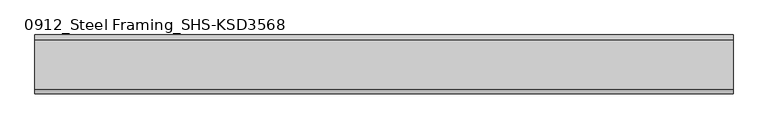
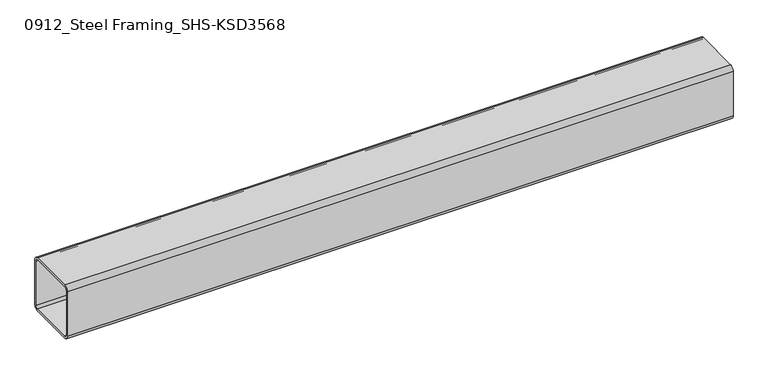
"""IFC4 building model written with IfcOpenShell, lengths in millimetres: beam geometry, 0912_Steel Framing_SHS-KSD3568 : H_SB_ASB_SHS-150x150x6."""

import ifcopenshell
import ifcopenshell.guid

model = None  # the IFC model being written
_history = None  # IfcOwnerHistory: only IFC2X3 demands one
_inside = {}  # id of a spatial element -> (the spatial element, [elements in it])
_under = {}  # id of a project, library or spatial element -> (it, [spatial elements below it])
_declared = {}  # id of a project -> (the project, [libraries it declares])
_typed = {}  # id of a type object -> (the type object, [elements of that type])
_made_of = {}  # id of a material, layer set ... -> (it, [elements and type objects made of it])


def new_model(schema):
    """Start an empty IFC model of exactly this schema.

    Asked for "IFC4X3", IfcOpenShell would pick the latest addendum, in which some entities
    have other attributes; the version numbers below select the first issue.
    IFC2X3 requires an IfcOwnerHistory on every rooted entity: one is made here for all.
    """
    global model, _history
    if schema == "IFC4X3":
        model = ifcopenshell.file(schema_version=(4, 3, 0, 0))
    else:
        model = ifcopenshell.file(schema=schema)
    _inside.clear()
    _under.clear()
    _declared.clear()
    _typed.clear()
    _made_of.clear()
    _history = None
    if model.schema == "IFC2X3":
        org = make("IfcOrganization", Name="unknown")
        user = make(
            "IfcPersonAndOrganization",
            ThePerson=make("IfcPerson", FamilyName="unknown"),
            TheOrganization=org,
        )
        app = make(
            "IfcApplication",
            ApplicationDeveloper=org,
            Version="unknown",
            ApplicationFullName="unknown",
            ApplicationIdentifier="unknown",
        )
        _history = make(
            "IfcOwnerHistory",
            OwningUser=user,
            OwningApplication=app,
            ChangeAction="ADDED",
            CreationDate=0,
        )
    return model


def make(cls, **values):
    """One entity of the class cls with the attributes given. An attribute that is None is left unset."""
    return model.create_entity(
        cls, **{name: value for name, value in values.items() if value is not None}
    )


def rooted(cls, **values):
    """An entity with a GlobalId (a new one), such as an element, a storey or a relation."""
    return make(cls, GlobalId=ifcopenshell.guid.new(), OwnerHistory=_history, **values)


def si_unit(unit_type, name, prefix=None):
    """IfcSIUnit, for example si_unit("LENGTHUNIT", "METRE", prefix="MILLI")."""
    return make("IfcSIUnit", UnitType=unit_type, Prefix=prefix, Name=name)


def assignment(units):
    """IfcUnitAssignment: the units of a project."""
    return None if units is None else make("IfcUnitAssignment", Units=units)


def point(xyz):
    """IfcCartesianPoint."""
    return None if xyz is None else make("IfcCartesianPoint", Coordinates=xyz)


def direction(xyz):
    """IfcDirection."""
    return None if xyz is None else make("IfcDirection", DirectionRatios=xyz)


def frame(location, z_axis=None, x_axis=None):
    """IfcAxis2Placement3D, a coordinate frame: its origin and axes. An axis left out is left unset."""
    return make(
        "IfcAxis2Placement3D",
        Location=point(location),
        Axis=direction(z_axis),
        RefDirection=direction(x_axis),
    )


def frame_2d(location, x_axis=None):
    """IfcAxis2Placement2D, a coordinate frame in the plane: its origin and x axis."""
    return make(
        "IfcAxis2Placement2D", Location=point(location), RefDirection=direction(x_axis)
    )


def origin():
    """The frame at (0, 0, 0) with its axes left unset."""
    return frame((0.0, 0.0, 0.0))


def place(relative_to, where):
    """IfcLocalPlacement: puts the frame where relative to a parent placement (None: the world)."""
    return make(
        "IfcLocalPlacement", PlacementRelTo=relative_to, RelativePlacement=where
    )


def context(
    kind, dimensions, precision=None, world=None, true_north=None, identifier=None
):
    """IfcGeometricRepresentationContext, for example the 3D "Model" context."""
    return make(
        "IfcGeometricRepresentationContext",
        ContextIdentifier=identifier,
        ContextType=kind,
        CoordinateSpaceDimension=dimensions,
        Precision=precision,
        WorldCoordinateSystem=world,
        TrueNorth=true_north,
    )


def project(units=None, contexts=None):
    """IfcProject with its units and contexts."""
    return rooted(
        "IfcProject",
        Name="project",
        RepresentationContexts=contexts,
        UnitsInContext=assignment(units),
    )


def spatial(cls, under=None, at=None, **own):
    """A site, building, storey or space (cls), placed at a placement, below another one or the project."""
    s = rooted(cls, ObjectPlacement=at, **own)
    if under is not None:
        _under.setdefault(under.id(), (under, []))[1].append(s)
    return s


def polyline(points):
    """IfcPolyline through the points."""
    return make("IfcPolyline", Points=[point(p) for p in points])


def circle_curve(where, radius):
    """IfcCircle in the frame where."""
    return make("IfcCircle", Position=where, Radius=radius)


def trimmed(basis, trim1, trim2, sense, master):
    """IfcTrimmedCurve: the piece of a basis curve between two trims."""
    return make(
        "IfcTrimmedCurve",
        BasisCurve=basis,
        Trim1=trim1,
        Trim2=trim2,
        SenseAgreement=sense,
        MasterRepresentation=master,
    )


def segment(curve, same_sense, transition):
    """IfcCompositeCurveSegment."""
    return make(
        "IfcCompositeCurveSegment",
        Transition=transition,
        SameSense=same_sense,
        ParentCurve=curve,
    )


def composite_curve(segments, self_intersect=None):
    """IfcCompositeCurve: segments joined end to end."""
    return make("IfcCompositeCurve", Segments=segments, SelfIntersect=self_intersect)


def outline(outer, holes=None, kind="AREA"):
    """IfcArbitraryClosedProfileDef: a profile drawn as a closed curve; with holes, ...WithVoids."""
    if holes is None:
        return make("IfcArbitraryClosedProfileDef", ProfileType=kind, OuterCurve=outer)
    return make(
        "IfcArbitraryProfileDefWithVoids",
        ProfileType=kind,
        OuterCurve=outer,
        InnerCurves=holes,
    )


def extrude(swept, where, along, depth):
    """IfcExtrudedAreaSolid: the profile swept, set in the frame where, extruded along a direction by depth."""
    return make(
        "IfcExtrudedAreaSolid",
        SweptArea=swept,
        Position=where,
        ExtrudedDirection=direction(along),
        Depth=depth,
    )


def shape(context_of_items, identifier, shape_type, items):
    """IfcShapeRepresentation: the items that make up one representation, for example the "Body"."""
    return make(
        "IfcShapeRepresentation",
        ContextOfItems=context_of_items,
        RepresentationIdentifier=identifier,
        RepresentationType=shape_type,
        Items=items,
    )


def source(mapping_origin, context_of_items, identifier, shape_type, items):
    """IfcRepresentationMap: a shape defined once, which mapped items show again and again."""
    return make(
        "IfcRepresentationMap",
        MappingOrigin=mapping_origin,
        MappedRepresentation=shape(context_of_items, identifier, shape_type, items),
    )


def transform(
    local_origin,
    x_axis=None,
    y_axis=None,
    z_axis=None,
    scale=None,
    scale2=None,
    scale3=None,
    uniform=True,
):
    """IfcCartesianTransformationOperator3D, or its non-uniform kind. x_axis, y_axis, z_axis: its Axis1, 2, 3."""
    if uniform:
        return make(
            "IfcCartesianTransformationOperator3D",
            Axis1=direction(x_axis),
            Axis2=direction(y_axis),
            LocalOrigin=point(local_origin),
            Scale=scale,
            Axis3=direction(z_axis),
        )
    return make(
        "IfcCartesianTransformationOperator3DnonUniform",
        Axis1=direction(x_axis),
        Axis2=direction(y_axis),
        LocalOrigin=point(local_origin),
        Scale=scale,
        Axis3=direction(z_axis),
        Scale2=scale2,
        Scale3=scale3,
    )


def mapped(mapping_source, mapping_target):
    """IfcMappedItem: shows the shape of a source again, moved by a transform."""
    return make(
        "IfcMappedItem", MappingSource=mapping_source, MappingTarget=mapping_target
    )


def made_of(thing, what):
    """Note that an element or type object is made of a material, layer set ...; save() writes the relation."""
    if what is not None:
        _made_of.setdefault(what.id(), (what, []))[1].append(thing)
    return thing


def element(
    cls,
    number,
    at=None,
    inside=None,
    cuts=None,
    type_object=None,
    material=None,
    context=None,
    identifier="Body",
    shape_type=None,
    held_by="IfcProductDefinitionShape",
    body=None,
    shapes=None,
    **own,
):
    """One element of the class cls, such as IfcWall. Its Tag is "e" and its number.

    at: its placement. inside: the storey or other place that contains it. cuts: it is an
    opening in that element (IfcRelVoidsElement). A single representation is given by context,
    identifier, shape_type and body (its items); several are given by shapes. held_by: the class
    of the entity that holds the representations. save() writes the other relations.
    """
    e = rooted(cls, Tag="e%d" % number, ObjectPlacement=at, **own)
    if body is not None:
        shapes = [shape(context, identifier, shape_type, body)]
    if shapes is not None:
        e.Representation = make(held_by, Representations=shapes)
    if inside is not None:
        _inside.setdefault(inside.id(), (inside, []))[1].append(e)
    if cuts is not None:
        rooted(
            "IfcRelVoidsElement", RelatingBuildingElement=cuts, RelatedOpeningElement=e
        )
    if type_object is not None:
        _typed.setdefault(type_object.id(), (type_object, []))[1].append(e)
    return made_of(e, material)


def aggregate(whole, parts):
    """IfcRelAggregates: a whole, such as a stair, and the parts it consists of."""
    return rooted("IfcRelAggregates", RelatingObject=whole, RelatedObjects=parts)


def save(model, path):
    """Write the relations noted so far, then the file.

    IfcRelAggregates (storeys below a building ...), IfcRelContainedInSpatialStructure (elements
    in a storey), IfcRelDefinesByType, IfcRelAssociatesMaterial and IfcRelDeclares: one each for
    every whole, place, type object, material and project.
    """
    for whole, parts in _under.values():
        aggregate(whole, parts)
    for where, things in _inside.values():
        rooted(
            "IfcRelContainedInSpatialStructure",
            RelatedElements=things,
            RelatingStructure=where,
        )
    for kind, things in _typed.values():
        rooted("IfcRelDefinesByType", RelatedObjects=things, RelatingType=kind)
    for what, things in _made_of.values():
        rooted("IfcRelAssociatesMaterial", RelatedObjects=things, RelatingMaterial=what)
    for by, libraries in _declared.values():
        rooted("IfcRelDeclares", RelatingContext=by, RelatedDefinitions=libraries)
    model.write(path)


def beam_0912_steel_framing_shs_ksd3568_3ef75c45(model_context):
    return source(origin(), model_context, "Body", "SweptSolid", [
        extrude(outline(composite_curve([segment(polyline([(75.0, 63.0), (75.0, -63.0)]), True, "CONTINUOUS"), segment(trimmed(circle_curve(frame_2d((63.0, -63.0)), 12.0), [point((75.0, -63.0))], [point((63.0, -75.0))], False, "CARTESIAN"), True, "CONTINUOUS"), segment(polyline([(63.0, -75.0), (-63.0, -75.0)]), True, "CONTINUOUS"), segment(trimmed(circle_curve(frame_2d((-63.0, -63.0)), 12.0), [point((-63.0, -75.0))], [point((-75.0, -63.0))], False, "CARTESIAN"), True, "CONTINUOUS"), segment(polyline([(-75.0, -63.0), (-75.0, 63.0)]), True, "CONTINUOUS"), segment(trimmed(circle_curve(frame_2d((-63.0, 63.0)), 12.0), [point((-75.0, 63.0))], [point((-63.0, 75.0))], False, "CARTESIAN"), True, "CONTINUOUS"), segment(polyline([(-63.0, 75.0), (63.0, 75.0)]), True, "CONTINUOUS"), segment(trimmed(circle_curve(frame_2d((63.0, 63.0)), 12.0), [point((63.0, 75.0))], [point((75.0, 63.0))], False, "CARTESIAN"), True, "CONTINUOUS")], self_intersect=False), holes=[composite_curve([segment(trimmed(circle_curve(frame_2d((-63.0, 63.0)), 6.0), [point((-63.0, 69.0))], [point((-69.0, 63.0))], True, "CARTESIAN"), True, "CONTINUOUS"), segment(polyline([(-69.0, 63.0), (-69.0, -63.0)]), True, "CONTINUOUS"), segment(trimmed(circle_curve(frame_2d((-63.0, -63.0)), 6.0), [point((-69.0, -63.0))], [point((-63.0, -69.0))], True, "CARTESIAN"), True, "CONTINUOUS"), segment(polyline([(-63.0, -69.0), (63.0, -69.0)]), True, "CONTINUOUS"), segment(trimmed(circle_curve(frame_2d((63.0, -63.0)), 6.0), [point((63.0, -69.0))], [point((69.0, -63.0))], True, "CARTESIAN"), True, "CONTINUOUS"), segment(polyline([(69.0, -63.0), (69.0, 63.0)]), True, "CONTINUOUS"), segment(trimmed(circle_curve(frame_2d((63.0, 63.0)), 6.0), [point((69.0, 63.0))], [point((63.0, 69.0))], True, "CARTESIAN"), True, "CONTINUOUS"), segment(polyline([(63.0, 69.0), (-63.0, 69.0)]), True, "CONTINUOUS")], self_intersect=False)]), frame((-890.0, 0.0, 0.0), z_axis=(1.0, 0.0, 0.0), x_axis=(0.0, 1.0, 0.0)), (0.0, 0.0, 1.0), 1780.0),
    ])


if __name__ == "__main__":
    model = new_model("IFC4")
    model_context = context("Model", 3, world=origin())
    ifc_project = project(units=[si_unit("LENGTHUNIT", "METRE", prefix="MILLI")], contexts=[model_context])
    site = spatial("IfcSite", under=ifc_project)
    building = spatial("IfcBuilding", under=site)
    placement = place(None, origin())
    beam_0912_steel_framing_shs_ksd3568_shape = beam_0912_steel_framing_shs_ksd3568_3ef75c45(model_context)
    element("IfcBeam", 1, ObjectType="0912_Steel Framing_SHS-KSD3568 : H_SB_ASB_SHS-150x150x6", at=placement, inside=building, context=model_context, shape_type="MappedRepresentation", body=[
        mapped(beam_0912_steel_framing_shs_ksd3568_shape, transform((0.0, 0.0, 0.0), x_axis=(1.0, 0.0, 0.0), y_axis=(0.0, 1.0, 0.0), z_axis=(0.0, 0.0, 1.0))),
    ])
    save(model, "model.ifc")

# Revit data of these elements
# Type "0912_Steel Framing_SHS-KSD3568 : H_SB_ASB_SHS-150x150x6"
#   H_WM Code_1 = "S01AA002-00001 | Main Steel Structure Fabrication Work | Shelter/Building | Medium Steel - Standard (90KG/M>Weight≥30KG/M) | Material: (   )"
#   H_WM Code_2 = "S03AA028-00001 | Main Steel Structure Erection Work | Shelter/Building | Medium Steel (90KG/M>Weight≥30KG/M) | Material: (   )"
#   H_WM Code_3 = "S01AA010-00001 | Main Steel Structure Fabrication Work | Shelter/Building | Steel Painting/Coating | for Non-Fireproofed Steel Surface, Surface Preparation, Primer, Second & Final Coat | Material: (   )"
#   H_Q'ty Cal Type Tag = "SB-Q2"
#   Perimeter = 0.60 m²/m
#   Nominal Weight = 26.40 kgf/m
#   Length [instance default] = 1.0000 m
#   b = 0.1500 m
#   h = 0.1500 m
#   tr = 0.0120 m
#   t = 0.0060 m
#   A = 28.36 m²
#   Structural Material [instance default] = Steel, 45-345
# Element 1 (IfcBeam, "0912_Steel Framing_SHS-KSD3568 : H_SB_ASB_SHS-150x150x6")
#   Structural Material = none
# Materials
#   "Steel, 45-345": class "Metal", colour RGB 189 187 185, transparency 0, Description = "Steel 345 MPa", Cost = 0
